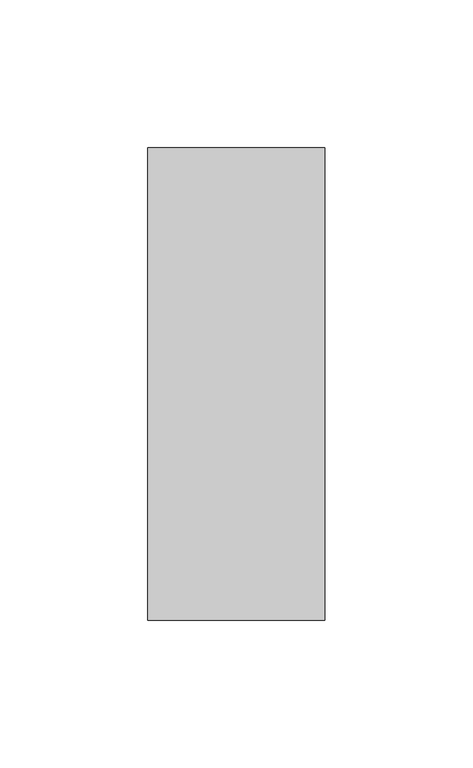
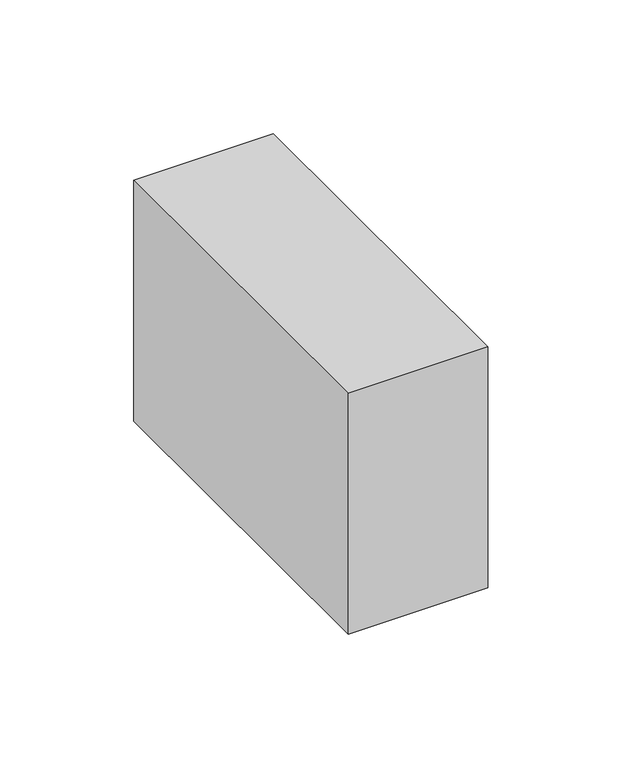
"""IFC4 building model written with IfcOpenShell, lengths in millimetres: column geometry, Madeira de lei-Coluna : Pontalete 6X16cm."""

from ifc_helpers import new_model, si_unit, frame, origin, place, context, project, spatial, polyline, outline, extrude, source, transform, mapped, element, save


def column_00c463e4(model_context):
    return source(origin(), model_context, "Body", "SweptSolid", [
        extrude(outline(polyline([(30.0, 80.0), (30.0, -80.0), (-30.0, -80.0), (-30.0, 80.0), (30.0, 80.0)])), frame((0.0, 0.0, 3110.0), z_axis=(0.0, 0.0, 1.0), x_axis=(1.0, 0.0, 0.0)), (0.0, 0.0, 1.0), 109.8),
    ])


if __name__ == "__main__":
    model = new_model("IFC4")
    model_context = context("Model", 3, world=origin())
    ifc_project = project(units=[si_unit("LENGTHUNIT", "METRE", prefix="MILLI")], contexts=[model_context])
    site = spatial("IfcSite", under=ifc_project)
    building = spatial("IfcBuilding", under=site)
    placement = place(None, origin())
    column_shape = column_00c463e4(model_context)
    element("IfcColumn", 1, ObjectType="Madeira de lei-Coluna : Pontalete 6X16cm", at=placement, inside=building, context=model_context, shape_type="MappedRepresentation", body=[
        mapped(column_shape, transform((0.0, 0.0, 0.0), x_axis=(1.0, 0.0, 0.0), y_axis=(0.0, 1.0, 0.0), z_axis=(0.0, 0.0, 1.0))),
    ])
    save(model, "model.ifc")

# Revit data of these elements
# Type "Madeira de lei-Coluna : Pontalete 6X16cm"
#   A = 0.01952 m²
#   b = 0.06 m
#   d = 0.16 m
#   Structural Material [instance default] = none
#   Assembly Code = ""
# Element 1 (IfcColumn, "Madeira de lei-Coluna : Pontalete 6X16cm")
#   Structural Material = .MADEIRAMENTO
#   Materials on its faces: ".MADEIRAMENTO"
# Materials
#   ".MADEIRAMENTO": class ".CC_MADEIRAS", colour RGB 212 179 113, transparency 0, Cost = 0
